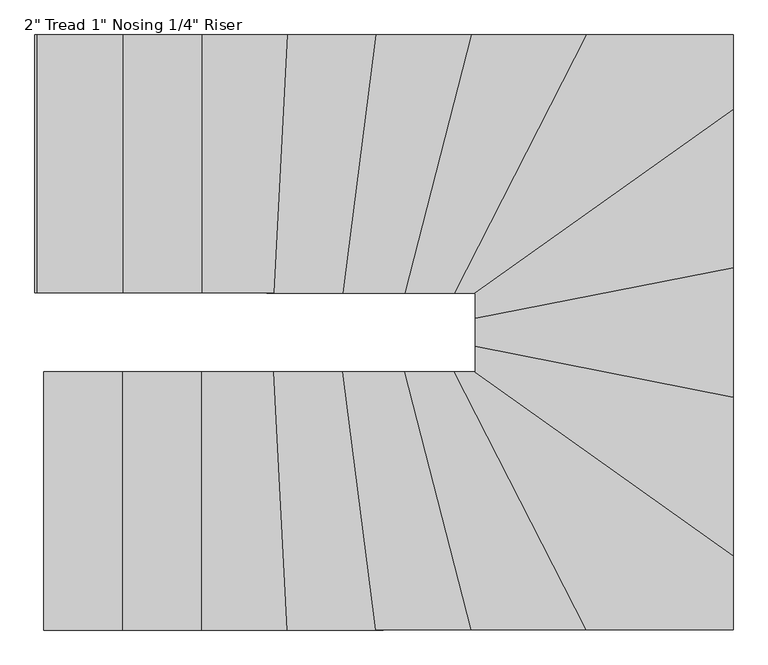
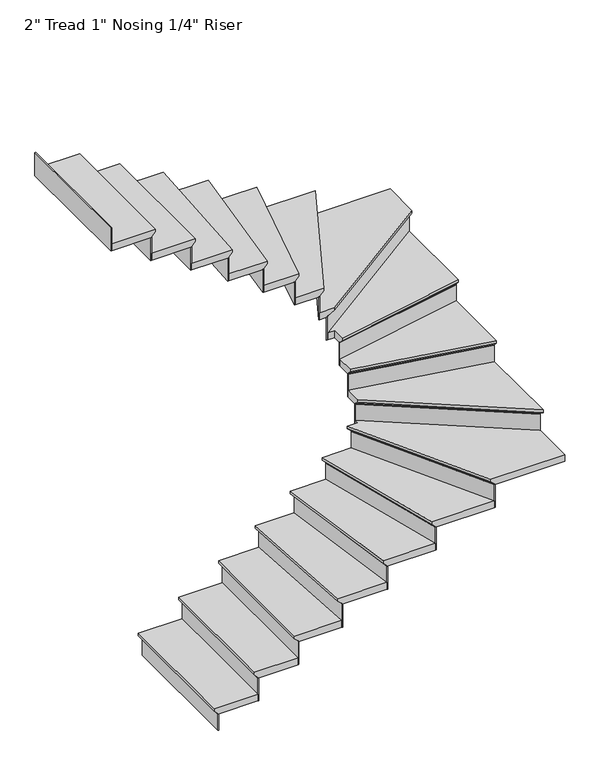
"""IFC4 building model written with IfcOpenShell, lengths in millimetres: stair flight geometry."""

from ifc_helpers import new_model, si_unit, origin, place, context, project, spatial, faceted_brep, source, transform, mapped, element, save


def stair_flight_c1eb027c(model_context):
    return source(origin(), model_context, "Body", "Brep", [
        faceted_brep([(-16321.7832832, 2938.4294183, 150.2833333), (-16321.7832832, 2938.4294183, 169.3333333), (-16321.7832832, 3852.8294183, 169.3333333), (-16321.7832832, 3852.8294183, 150.2833333), (-16296.3832832, 2938.4294183, 124.8833333), (-16296.3832832, 3852.8294183, 124.8833333), (-16016.9832832, 2938.4294183, 169.3333333), (-16016.9832832, 3852.8294183, 169.3333333), (-16296.3832832, 3852.8294183, 118.5333333), (-16016.9832832, 3852.8294183, 118.5333333), (-16016.9832832, 2938.4294183, 118.5333333), (-16296.3832832, 2938.4294183, 118.5333333)], [[[0, 1, 2, 3]], [[4, 0, 3, 5]], [[2, 1, 6, 7]], [[8, 9, 10, 11]], [[2, 7, 9, 8, 5, 3]], [[8, 11, 4, 5]], [[6, 1, 0, 4, 11, 10]], [[7, 6, 10, 9]]]),
        faceted_brep([(-16296.3832832, 2938.4294183, 118.5333333), (-16296.3832832, 2938.4294183, 0.0), (-16290.0332832, 2938.4294183, 0.0), (-16290.0332832, 2938.4294183, 118.5333333), (-16296.3832832, 3852.8294183, 118.5333333), (-16290.0332832, 3852.8294183, 118.5333333), (-16290.0332832, 3852.8294183, 0.0), (-16296.3832832, 3852.8294183, 0.0)], [[[0, 1, 2, 3]], [[4, 5, 6, 7]], [[1, 0, 4, 7]], [[2, 1, 7, 6]], [[3, 2, 6, 5]], [[0, 3, 5, 4]]]),
        faceted_brep([(-16016.9832832, 2938.4294183, 287.8666667), (-16016.9832832, 2938.4294183, 118.5333333), (-16010.6332832, 2938.4294183, 118.5333333), (-16010.6332832, 2938.4294183, 287.8666667), (-16016.9832832, 3852.8294183, 287.8666667), (-16010.6332832, 3852.8294183, 287.8666667), (-16010.6332832, 3852.8294183, 118.5333333), (-16016.9832832, 3852.8294183, 118.5333333)], [[[0, 1, 2, 3]], [[4, 5, 6, 7]], [[1, 0, 4, 7]], [[2, 1, 7, 6]], [[3, 2, 6, 5]], [[0, 3, 5, 4]]]),
        faceted_brep([(-16042.3832832, 3852.8294183, 338.6666667), (-16042.3832832, 2938.4294183, 338.6666667), (-15737.5832832, 2938.4294183, 338.6666667), (-15737.5832832, 3852.8294183, 338.6666667), (-16016.9832832, 3852.8294183, 287.8666667), (-15737.5832832, 3852.8294183, 287.8666667), (-15737.5832832, 2938.4294183, 287.8666667), (-16016.9832832, 2938.4294183, 287.8666667), (-16016.9832832, 3852.8294183, 294.2166667), (-16042.3832832, 3852.8294183, 319.6166667), (-16016.9832832, 2938.4294183, 294.2166667), (-16042.3832832, 2938.4294183, 319.6166667)], [[[0, 1, 2, 3]], [[4, 5, 6, 7]], [[0, 3, 5, 4, 8, 9]], [[4, 7, 10, 8]], [[2, 1, 11, 10, 7, 6]], [[3, 2, 6, 5]], [[11, 1, 0, 9]], [[10, 11, 9, 8]]]),
        faceted_brep([(-15737.5832832, 2938.4294183, 457.2), (-15737.5832832, 2938.4294183, 287.8666667), (-15731.2332832, 2938.4294183, 287.8666667), (-15731.2332832, 2938.4294183, 457.2), (-15737.5832832, 3852.8294183, 457.2), (-15731.2332832, 3852.8294183, 457.2), (-15731.2332832, 3852.8294183, 287.8666667), (-15737.5832832, 3852.8294183, 287.8666667)], [[[0, 1, 2, 3]], [[4, 5, 6, 7]], [[1, 0, 4, 7]], [[2, 1, 7, 6]], [[3, 2, 6, 5]], [[0, 3, 5, 4]]]),
        faceted_brep([(-15762.9832832, 3852.8294183, 508.0), (-15762.9832832, 2938.4294183, 508.0), (-15434.3818513, 2938.4294183, 508.0), (-15481.9161218, 3852.8294183, 508.0), (-15737.5832832, 3852.8294183, 457.2), (-15481.9161218, 3852.8294183, 457.2), (-15434.3818513, 2938.4294183, 457.2), (-15737.5832832, 2938.4294183, 457.2), (-15737.5832832, 3852.8294183, 463.55), (-15762.9832832, 3852.8294183, 488.95), (-15737.5832832, 2938.4294183, 463.55), (-15762.9832832, 2938.4294183, 488.95)], [[[0, 1, 2, 3]], [[4, 5, 6, 7]], [[0, 3, 5, 4, 8, 9]], [[4, 7, 10, 8]], [[2, 1, 11, 10, 7, 6]], [[3, 2, 6, 5]], [[11, 1, 0, 9]], [[10, 11, 9, 8]]]),
        faceted_brep([(-15434.3818513, 2938.4294183, 626.5333333), (-15434.3818513, 2938.4294183, 457.2), (-15428.0232772, 2938.4294183, 457.2), (-15428.0232772, 2938.4294183, 626.5333333), (-15481.9161218, 3852.8294183, 626.5333333), (-15475.5575476, 3852.8294183, 626.5333333), (-15475.5575476, 3852.8294183, 457.2), (-15481.9161218, 3852.8294183, 457.2)], [[[0, 1, 2, 3]], [[4, 5, 6, 7]], [[1, 0, 4, 7]], [[2, 1, 7, 6]], [[3, 2, 6, 5]], [[0, 3, 5, 4]]]),
        faceted_brep([(-15507.3504184, 3852.8294183, 677.3333333), (-15459.816148, 2938.4294183, 677.3333333), (-15119.3933703, 2938.4294183, 677.3333333), (-15237.7494219, 3852.8294183, 677.3333333), (-15481.9161218, 3852.8294183, 626.5333333), (-15237.7494219, 3852.8294183, 626.5333333), (-15119.3933703, 2938.4294183, 626.5333333), (-15434.3818513, 2938.4294183, 626.5333333), (-15481.9161218, 3852.8294183, 632.8833333), (-15507.3504184, 3852.8294183, 658.2833333), (-15434.3818513, 2938.4294183, 632.8833333), (-15459.816148, 2938.4294183, 658.2833333)], [[[0, 1, 2, 3]], [[4, 5, 6, 7]], [[0, 3, 5, 4, 8, 9]], [[4, 7, 10, 8]], [[2, 1, 11, 10, 7, 6]], [[3, 2, 6, 5]], [[11, 1, 0, 9]], [[10, 11, 9, 8]]]),
        faceted_brep([(-15119.3933703, 2938.4294183, 795.8666667), (-15119.3933703, 2938.4294183, 626.5333333), (-15112.9903985, 2938.4294183, 626.5333333), (-15112.9903985, 2938.4294183, 795.8666667), (-15237.7494219, 3852.8294183, 795.8666667), (-15231.3464501, 3852.8294183, 795.8666667), (-15231.3464501, 3852.8294183, 626.5333333), (-15237.7494219, 3852.8294183, 626.5333333)], [[[0, 1, 2, 3]], [[4, 5, 6, 7]], [[1, 0, 4, 7]], [[2, 1, 7, 6]], [[3, 2, 6, 5]], [[0, 3, 5, 4]]]),
        faceted_brep([(-15263.361309, 3852.8294183, 846.6666667), (-15145.0052574, 2938.4294183, 846.6666667), (-14780.991752, 2938.4294183, 846.6666667), (-15016.1221995, 3852.8294183, 846.6666667), (-15237.7494219, 3852.8294183, 795.8666667), (-15016.1221995, 3852.8294183, 795.8666667), (-14780.991752, 2938.4294183, 795.8666667), (-15119.3933703, 2938.4294183, 795.8666667), (-15237.7494219, 3852.8294183, 802.2166667), (-15263.361309, 3852.8294183, 827.6166667), (-15119.3933703, 2938.4294183, 802.2166667), (-15145.0052574, 2938.4294183, 827.6166667)], [[[0, 1, 2, 3]], [[4, 5, 6, 7]], [[0, 3, 5, 4, 8, 9]], [[4, 7, 10, 8]], [[2, 1, 11, 10, 7, 6]], [[3, 2, 6, 5]], [[11, 1, 0, 9]], [[10, 11, 9, 8]]]),
        faceted_brep([(-14780.991752, 2938.4294183, 965.2), (-14780.991752, 2938.4294183, 795.8666667), (-14774.4351752, 2938.4294183, 795.8666667), (-14774.4351752, 2938.4294183, 965.2), (-15016.1221995, 3852.8294183, 965.2), (-15009.5656226, 3852.8294183, 965.2), (-15009.5656226, 3852.8294183, 795.8666667), (-15016.1221995, 3852.8294183, 795.8666667)], [[[0, 1, 2, 3]], [[4, 5, 6, 7]], [[1, 0, 4, 7]], [[2, 1, 7, 6]], [[3, 2, 6, 5]], [[0, 3, 5, 4]]]),
        faceted_brep([(-15042.3485069, 3852.8294183, 1016.0), (-14807.2180595, 2938.4294183, 1016.0), (-14370.950942, 2938.4294183, 1016.0), (-14839.7755634, 3852.8294183, 1016.0), (-15016.1221995, 3852.8294183, 965.2), (-14839.7755634, 3852.8294183, 965.2), (-14370.950942, 2938.4294183, 965.2), (-14780.991752, 2938.4294183, 965.2), (-15016.1221995, 3852.8294183, 971.55), (-15042.3485069, 3852.8294183, 996.95), (-14780.991752, 2938.4294183, 971.55), (-14807.2180595, 2938.4294183, 996.95)], [[[0, 1, 2, 3]], [[4, 5, 6, 7]], [[0, 3, 5, 4, 8, 9]], [[4, 7, 10, 8]], [[2, 1, 11, 10, 7, 6]], [[3, 2, 6, 5]], [[11, 1, 0, 9]], [[10, 11, 9, 8]]]),
        faceted_brep([(-14370.950942, 2938.4294183, 1134.5333333), (-14370.950942, 2938.4294183, 965.2), (-14363.8149589, 2938.4294183, 965.2), (-14363.8149589, 2938.4294183, 1134.5333333), (-14839.7755634, 3852.8294183, 1134.5333333), (-14832.6395802, 3852.8294183, 1134.5333333), (-14832.6395802, 3852.8294183, 965.2), (-14839.7755634, 3852.8294183, 965.2)], [[[0, 1, 2, 3]], [[4, 5, 6, 7]], [[1, 0, 4, 7]], [[2, 1, 7, 6]], [[3, 2, 6, 5]], [[0, 3, 5, 4]]]),
        faceted_brep([(-14794.0515914, 3882.3845011, 1185.3333333), (-14794.0515914, 3852.8294183, 1185.3333333), (-14868.3194959, 3852.8294183, 1185.3333333), (-14399.4948746, 2938.4294183, 1185.3333333), (-13879.6515914, 2938.4294183, 1185.3333333), (-13879.6515914, 3232.110552, 1185.3333333), (-14794.0515914, 3852.8294183, 1134.5333333), (-14794.0515914, 3882.3845011, 1134.5333333), (-13879.6515914, 3232.110552, 1134.5333333), (-13879.6515914, 2938.4294183, 1134.5333333), (-14370.950942, 2938.4294183, 1134.5333333), (-14839.7755634, 3852.8294183, 1134.5333333), (-14839.7755634, 3852.8294183, 1140.8833333), (-14868.3194959, 3852.8294183, 1166.2833333), (-14370.950942, 2938.4294183, 1140.8833333), (-14399.4948746, 2938.4294183, 1166.2833333)], [[[0, 1, 2, 3, 4, 5]], [[6, 7, 8, 9, 10, 11]], [[1, 0, 7, 6]], [[2, 1, 6, 11, 12, 13]], [[11, 10, 14, 12]], [[4, 3, 15, 14, 10, 9]], [[5, 4, 9, 8]], [[0, 5, 8, 7]], [[15, 3, 2, 13]], [[14, 15, 13, 12]]]),
        faceted_brep([(-13879.6515914, 3232.110552, 1303.8666667), (-13879.6515914, 3232.110552, 1134.5333333), (-13879.6515914, 3239.9025268, 1134.5333333), (-13879.6515914, 3239.9025268, 1303.8666667), (-14794.0515914, 3882.3845011, 1303.8666667), (-14794.0515914, 3890.1764759, 1303.8666667), (-14794.0515914, 3890.1764759, 1134.5333333), (-14794.0515914, 3882.3845011, 1134.5333333)], [[[0, 1, 2, 3]], [[4, 5, 6, 7]], [[1, 0, 4, 7]], [[2, 1, 7, 6]], [[3, 2, 6, 5]], [[0, 3, 5, 4]]]),
        faceted_brep([(-14794.0515914, 3851.2166019, 1354.6666667), (-13879.6515914, 3200.9426528, 1354.6666667), (-13879.6515914, 3788.5977319, 1354.6666667), (-14794.0515914, 3968.8385882, 1354.6666667), (-14794.0515914, 3882.3845011, 1303.8666667), (-14794.0515914, 3968.8385882, 1303.8666667), (-13879.6515914, 3788.5977319, 1303.8666667), (-13879.6515914, 3232.110552, 1303.8666667), (-14794.0515914, 3882.3845011, 1310.2166667), (-14794.0515914, 3851.2166019, 1335.6166667), (-13879.6515914, 3232.110552, 1310.2166667), (-13879.6515914, 3200.9426528, 1335.6166667)], [[[0, 1, 2, 3]], [[4, 5, 6, 7]], [[0, 3, 5, 4, 8, 9]], [[4, 7, 10, 8]], [[3, 2, 6, 5]], [[11, 1, 0, 9]], [[10, 11, 9, 8]], [[2, 1, 11, 10, 7, 6]]]),
        faceted_brep([(-13879.6515914, 3788.5977319, 1473.2), (-13879.6515914, 3788.5977319, 1303.8666667), (-13879.6515914, 3795.0699173, 1303.8666667), (-13879.6515914, 3795.0699173, 1473.2), (-14794.0515914, 3968.8385882, 1473.2), (-14794.0515914, 3975.3107736, 1473.2), (-14794.0515914, 3975.3107736, 1303.8666667), (-14794.0515914, 3968.8385882, 1303.8666667)], [[[0, 1, 2, 3]], [[4, 5, 6, 7]], [[1, 0, 4, 7]], [[2, 1, 7, 6]], [[3, 2, 6, 5]], [[0, 3, 5, 4]]]),
        faceted_brep([(-14794.0515914, 3942.9498464, 1524.0), (-13879.6515914, 3762.7089901, 1524.0), (-13879.6515914, 4248.2385882, 1524.0), (-14794.0515914, 4067.9977319, 1524.0), (-14794.0515914, 3968.8385882, 1473.2), (-14794.0515914, 4067.9977319, 1473.2), (-13879.6515914, 4248.2385882, 1473.2), (-13879.6515914, 3788.5977319, 1473.2), (-14794.0515914, 3968.8385882, 1479.55), (-14794.0515914, 3942.9498464, 1504.95), (-13879.6515914, 3788.5977319, 1479.55), (-13879.6515914, 3762.7089901, 1504.95)], [[[0, 1, 2, 3]], [[4, 5, 6, 7]], [[0, 3, 5, 4, 8, 9]], [[4, 7, 10, 8]], [[2, 1, 11, 10, 7, 6]], [[3, 2, 6, 5]], [[11, 1, 0, 9]], [[10, 11, 9, 8]]]),
        faceted_brep([(-13879.6515914, 4248.2385882, 1642.5333333), (-13879.6515914, 4248.2385882, 1473.2), (-13879.6515914, 4254.7107736, 1473.2), (-13879.6515914, 4254.7107736, 1642.5333333), (-14794.0515914, 4067.9977319, 1642.5333333), (-14794.0515914, 4074.4699173, 1642.5333333), (-14794.0515914, 4074.4699173, 1473.2), (-14794.0515914, 4067.9977319, 1473.2)], [[[0, 1, 2, 3]], [[4, 5, 6, 7]], [[1, 0, 4, 7]], [[2, 1, 7, 6]], [[3, 2, 6, 5]], [[0, 3, 5, 4]]]),
        faceted_brep([(-14840.1470659, 4132.2294183, 1693.3333333), (-14794.0515914, 4132.2294183, 1693.3333333), (-14794.0515914, 4042.1089901, 1693.3333333), (-13879.6515914, 4222.3498464, 1693.3333333), (-13879.6515914, 4815.2840829, 1693.3333333), (-14794.0515914, 4132.2294183, 1642.5333333), (-14840.1470659, 4132.2294183, 1642.5333333), (-13879.6515914, 4815.2840829, 1642.5333333), (-13879.6515914, 4248.2385882, 1642.5333333), (-14794.0515914, 4067.9977319, 1642.5333333), (-13879.6515914, 4248.2385882, 1648.8833333), (-14794.0515914, 4067.9977319, 1648.8833333), (-13879.6515914, 4222.3498464, 1674.2833333), (-14794.0515914, 4042.1089901, 1674.2833333)], [[[0, 1, 2, 3, 4]], [[5, 6, 7, 8, 9]], [[1, 0, 6, 5]], [[9, 8, 10, 11]], [[4, 3, 12, 10, 8, 7]], [[0, 4, 7, 6]], [[12, 3, 2, 13]], [[10, 12, 13, 11]], [[2, 1, 5, 9, 11, 13]]]),
        faceted_brep([(-13879.6515914, 4815.2840829, 1811.8666667), (-13879.6515914, 4815.2840829, 1642.5333333), (-13879.6515914, 4823.0760577, 1642.5333333), (-13879.6515914, 4823.0760577, 1811.8666667), (-14840.1470659, 4132.2294183, 1811.8666667), (-14851.1039584, 4132.2294183, 1811.8666667), (-14851.1039584, 4132.2294183, 1642.5333333), (-14840.1470659, 4132.2294183, 1642.5333333)], [[[0, 1, 2, 3]], [[4, 5, 6, 7]], [[1, 0, 4, 7]], [[2, 1, 7, 6]], [[3, 2, 6, 5]], [[0, 3, 5, 4]]]),
        faceted_brep([(-14796.3194959, 4132.2294183, 1862.6666667), (-13879.6515914, 4784.1161838, 1862.6666667), (-13879.6515914, 5046.6294183, 1862.6666667), (-14428.0388071, 5046.6294183, 1862.6666667), (-14896.8634284, 4132.2294183, 1862.6666667), (-14840.1470659, 4132.2294183, 1811.8666667), (-14896.8634284, 4132.2294183, 1811.8666667), (-14428.0388071, 5046.6294183, 1811.8666667), (-13879.6515914, 5046.6294183, 1811.8666667), (-13879.6515914, 4815.2840829, 1811.8666667), (-14840.1470659, 4132.2294183, 1818.2166667), (-14796.3194959, 4132.2294183, 1843.6166667), (-13879.6515914, 4815.2840829, 1818.2166667), (-13879.6515914, 4784.1161838, 1843.6166667)], [[[0, 1, 2, 3, 4]], [[5, 6, 7, 8, 9]], [[0, 4, 6, 5, 10, 11]], [[5, 9, 12, 10]], [[2, 1, 13, 12, 9, 8]], [[4, 3, 7, 6]], [[13, 1, 0, 11]], [[12, 13, 11, 10]], [[3, 2, 8, 7]]]),
        faceted_brep([(-14428.0388071, 5046.6294183, 1981.2), (-14428.0388071, 5046.6294183, 1811.8666667), (-14435.1747902, 5046.6294183, 1811.8666667), (-14435.1747902, 5046.6294183, 1981.2), (-14896.8634284, 4132.2294183, 1981.2), (-14903.9994116, 4132.2294183, 1981.2), (-14903.9994116, 4132.2294183, 1811.8666667), (-14896.8634284, 4132.2294183, 1811.8666667)], [[[0, 1, 2, 3]], [[4, 5, 6, 7]], [[1, 0, 4, 7]], [[2, 1, 7, 6]], [[3, 2, 6, 5]], [[0, 3, 5, 4]]]),
        faceted_brep([(-14868.3194959, 4132.2294183, 2032.0), (-14399.4948746, 5046.6294183, 2032.0), (-14833.444367, 5046.6294183, 2032.0), (-15068.5748144, 4132.2294183, 2032.0), (-14896.8634284, 4132.2294183, 1981.2), (-15068.5748144, 4132.2294183, 1981.2), (-14833.444367, 5046.6294183, 1981.2), (-14428.0388071, 5046.6294183, 1981.2), (-14896.8634284, 4132.2294183, 1987.55), (-14868.3194959, 4132.2294183, 2012.95), (-14428.0388071, 5046.6294183, 1987.55), (-14399.4948746, 5046.6294183, 2012.95)], [[[0, 1, 2, 3]], [[4, 5, 6, 7]], [[0, 3, 5, 4, 8, 9]], [[4, 7, 10, 8]], [[2, 1, 11, 10, 7, 6]], [[3, 2, 6, 5]], [[11, 1, 0, 9]], [[10, 11, 9, 8]]]),
        faceted_brep([(-14833.444367, 5046.6294183, 2150.5333333), (-14833.444367, 5046.6294183, 1981.2), (-14840.0009438, 5046.6294183, 1981.2), (-14840.0009438, 5046.6294183, 2150.5333333), (-15068.5748144, 4132.2294183, 2150.5333333), (-15075.1313912, 4132.2294183, 2150.5333333), (-15075.1313912, 4132.2294183, 1981.2), (-15068.5748144, 4132.2294183, 1981.2)], [[[0, 1, 2, 3]], [[4, 5, 6, 7]], [[1, 0, 4, 7]], [[2, 1, 7, 6]], [[3, 2, 6, 5]], [[0, 3, 5, 4]]]),
        faceted_brep([(-15042.3485069, 4132.2294183, 2201.3333333), (-14807.2180595, 5046.6294183, 2201.3333333), (-15170.6171445, 5046.6294183, 2201.3333333), (-15288.9731962, 4132.2294183, 2201.3333333), (-15068.5748144, 4132.2294183, 2150.5333333), (-15288.9731962, 4132.2294183, 2150.5333333), (-15170.6171445, 5046.6294183, 2150.5333333), (-14833.444367, 5046.6294183, 2150.5333333), (-15068.5748144, 4132.2294183, 2156.8833333), (-15042.3485069, 4132.2294183, 2182.2833333), (-14833.444367, 5046.6294183, 2156.8833333), (-14807.2180595, 5046.6294183, 2182.2833333)], [[[0, 1, 2, 3]], [[4, 5, 6, 7]], [[0, 3, 5, 4, 8, 9]], [[4, 7, 10, 8]], [[2, 1, 11, 10, 7, 6]], [[3, 2, 6, 5]], [[11, 1, 0, 9]], [[10, 11, 9, 8]]]),
        faceted_brep([(-15170.6171445, 5046.6294183, 2319.8666667), (-15170.6171445, 5046.6294183, 2150.5333333), (-15177.0201163, 5046.6294183, 2150.5333333), (-15177.0201163, 5046.6294183, 2319.8666667), (-15288.9731962, 4132.2294183, 2319.8666667), (-15295.3761679, 4132.2294183, 2319.8666667), (-15295.3761679, 4132.2294183, 2150.5333333), (-15288.9731962, 4132.2294183, 2150.5333333)], [[[0, 1, 2, 3]], [[4, 5, 6, 7]], [[1, 0, 4, 7]], [[2, 1, 7, 6]], [[3, 2, 6, 5]], [[0, 3, 5, 4]]]),
        faceted_brep([(-15263.361309, 4132.2294183, 2370.6666667), (-15145.0052574, 5046.6294183, 2370.6666667), (-15485.2504447, 5046.6294183, 2370.6666667), (-15532.7847151, 4132.2294183, 2370.6666667), (-15288.9731962, 4132.2294183, 2319.8666667), (-15532.7847151, 4132.2294183, 2319.8666667), (-15485.2504447, 5046.6294183, 2319.8666667), (-15170.6171445, 5046.6294183, 2319.8666667), (-15288.9731962, 4132.2294183, 2326.2166667), (-15263.361309, 4132.2294183, 2351.6166667), (-15170.6171445, 5046.6294183, 2326.2166667), (-15145.0052574, 5046.6294183, 2351.6166667)], [[[0, 1, 2, 3]], [[4, 5, 6, 7]], [[0, 3, 5, 4, 8, 9]], [[4, 7, 10, 8]], [[2, 1, 11, 10, 7, 6]], [[3, 2, 6, 5]], [[11, 1, 0, 9]], [[10, 11, 9, 8]]]),
        faceted_brep([(-15485.2504447, 5046.6294183, 2489.2), (-15485.2504447, 5046.6294183, 2319.8666667), (-15491.6090188, 5046.6294183, 2319.8666667), (-15491.6090188, 5046.6294183, 2489.2), (-15532.7847151, 4132.2294183, 2489.2), (-15539.1432892, 4132.2294183, 2489.2), (-15539.1432892, 4132.2294183, 2319.8666667), (-15532.7847151, 4132.2294183, 2319.8666667)], [[[0, 1, 2, 3]], [[4, 5, 6, 7]], [[1, 0, 4, 7]], [[2, 1, 7, 6]], [[3, 2, 6, 5]], [[0, 3, 5, 4]]]),
        faceted_brep([(-15507.3504184, 4132.2294183, 2540.0), (-15459.816148, 5046.6294183, 2540.0), (-15788.3832832, 5046.6294183, 2540.0), (-15788.3832832, 4132.2294183, 2540.0), (-15532.7847151, 4132.2294183, 2489.2), (-15788.3832832, 4132.2294183, 2489.2), (-15788.3832832, 5046.6294183, 2489.2), (-15485.2504447, 5046.6294183, 2489.2), (-15532.7847151, 4132.2294183, 2495.55), (-15507.3504184, 4132.2294183, 2520.95), (-15485.2504447, 5046.6294183, 2495.55), (-15459.816148, 5046.6294183, 2520.95)], [[[0, 1, 2, 3]], [[4, 5, 6, 7]], [[0, 3, 5, 4, 8, 9]], [[4, 7, 10, 8]], [[2, 1, 11, 10, 7, 6]], [[3, 2, 6, 5]], [[11, 1, 0, 9]], [[10, 11, 9, 8]]]),
        faceted_brep([(-15788.3832832, 5046.6294183, 2658.5333333), (-15788.3832832, 5046.6294183, 2489.2), (-15794.7332832, 5046.6294183, 2489.2), (-15794.7332832, 5046.6294183, 2658.5333333), (-15788.3832832, 4132.2294183, 2658.5333333), (-15794.7332832, 4132.2294183, 2658.5333333), (-15794.7332832, 4132.2294183, 2489.2), (-15788.3832832, 4132.2294183, 2489.2)], [[[0, 1, 2, 3]], [[4, 5, 6, 7]], [[1, 0, 4, 7]], [[2, 1, 7, 6]], [[3, 2, 6, 5]], [[0, 3, 5, 4]]]),
        faceted_brep([(-15762.9832832, 4132.2294183, 2709.3333333), (-15762.9832832, 5046.6294183, 2709.3333333), (-16067.7832832, 5046.6294183, 2709.3333333), (-16067.7832832, 4132.2294183, 2709.3333333), (-15788.3832832, 4132.2294183, 2658.5333333), (-16067.7832832, 4132.2294183, 2658.5333333), (-16067.7832832, 5046.6294183, 2658.5333333), (-15788.3832832, 5046.6294183, 2658.5333333), (-15788.3832832, 4132.2294183, 2664.8833333), (-15762.9832832, 4132.2294183, 2690.2833333), (-15788.3832832, 5046.6294183, 2664.8833333), (-15762.9832832, 5046.6294183, 2690.2833333)], [[[0, 1, 2, 3]], [[4, 5, 6, 7]], [[0, 3, 5, 4, 8, 9]], [[4, 7, 10, 8]], [[2, 1, 11, 10, 7, 6]], [[3, 2, 6, 5]], [[11, 1, 0, 9]], [[10, 11, 9, 8]]]),
        faceted_brep([(-16067.7832832, 5046.6294183, 2827.8666667), (-16067.7832832, 5046.6294183, 2658.5333333), (-16074.1332832, 5046.6294183, 2658.5333333), (-16074.1332832, 5046.6294183, 2827.8666667), (-16067.7832832, 4132.2294183, 2827.8666667), (-16074.1332832, 4132.2294183, 2827.8666667), (-16074.1332832, 4132.2294183, 2658.5333333), (-16067.7832832, 4132.2294183, 2658.5333333)], [[[0, 1, 2, 3]], [[4, 5, 6, 7]], [[1, 0, 4, 7]], [[2, 1, 7, 6]], [[3, 2, 6, 5]], [[0, 3, 5, 4]]]),
        faceted_brep([(-16347.1832832, 5046.6294183, 2997.2), (-16347.1832832, 5046.6294183, 2827.8666667), (-16353.5332832, 5046.6294183, 2827.8666667), (-16353.5332832, 5046.6294183, 2997.2), (-16347.1832832, 4132.2294183, 2997.2), (-16353.5332832, 4132.2294183, 2997.2), (-16353.5332832, 4132.2294183, 2827.8666667), (-16347.1832832, 4132.2294183, 2827.8666667)], [[[0, 1, 2, 3]], [[4, 5, 6, 7]], [[1, 0, 4, 7]], [[2, 1, 7, 6]], [[3, 2, 6, 5]], [[0, 3, 5, 4]]]),
        faceted_brep([(-16042.3832832, 4132.2294183, 2878.6666667), (-16042.3832832, 5046.6294183, 2878.6666667), (-16347.1832832, 5046.6294183, 2878.6666667), (-16347.1832832, 4132.2294183, 2878.6666667), (-16067.7832832, 4132.2294183, 2827.8666667), (-16347.1832832, 4132.2294183, 2827.8666667), (-16347.1832832, 5046.6294183, 2827.8666667), (-16067.7832832, 5046.6294183, 2827.8666667), (-16067.7832832, 4132.2294183, 2834.2166667), (-16042.3832832, 4132.2294183, 2859.6166667), (-16067.7832832, 5046.6294183, 2834.2166667), (-16042.3832832, 5046.6294183, 2859.6166667)], [[[0, 1, 2, 3]], [[4, 5, 6, 7]], [[0, 3, 5, 4, 8, 9]], [[4, 7, 10, 8]], [[2, 1, 11, 10, 7, 6]], [[3, 2, 6, 5]], [[11, 1, 0, 9]], [[10, 11, 9, 8]]]),
    ])


if __name__ == "__main__":
    model = new_model("IFC4")
    model_context = context("Model", 3, world=origin())
    ifc_project = project(units=[si_unit("LENGTHUNIT", "METRE", prefix="MILLI")], contexts=[model_context])
    site = spatial("IfcSite", under=ifc_project)
    building = spatial("IfcBuilding", under=site)
    placement = place(None, origin())
    stair_flight_shape = stair_flight_c1eb027c(model_context)
    element("IfcStairFlight", 1, ObjectType="2\" Tread 1\" Nosing 1/4\" Riser", at=placement, inside=building, context=model_context, shape_type="MappedRepresentation", body=[
        mapped(stair_flight_shape, transform((0.0, 0.0, 0.0), x_axis=(1.0, 0.0, 0.0), y_axis=(0.0, 1.0, 0.0), z_axis=(0.0, 0.0, 1.0))),
    ])
    save(model, "model.ifc")
